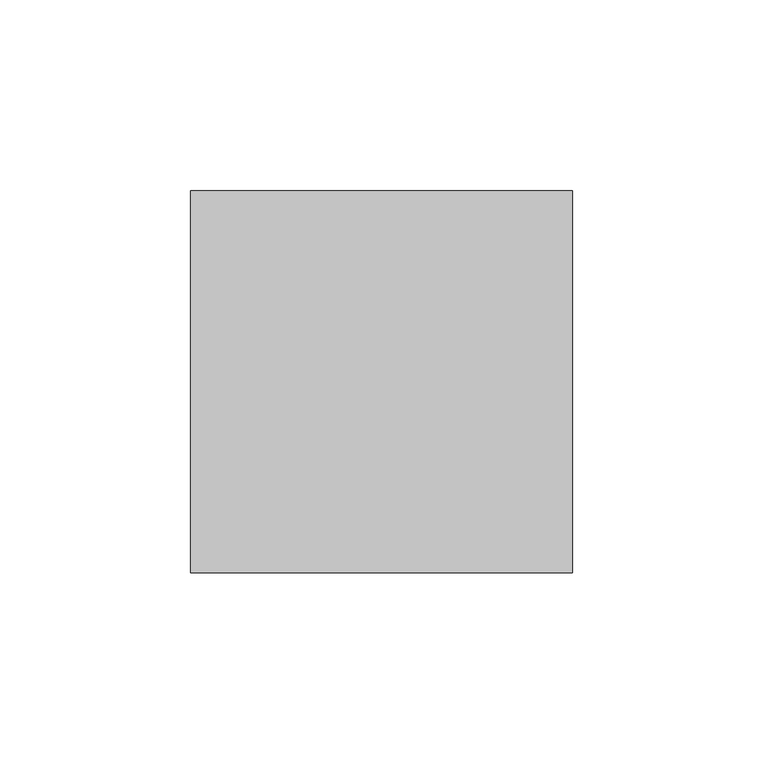
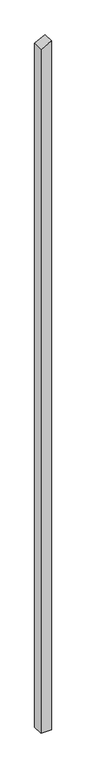
"""IFC4 building model written with IfcOpenShell, lengths in millimetres: column geometry, Holzstütze 159756 : Holzstütze 159756."""

from ifc_helpers import new_model, si_unit, frame, origin, place, context, project, spatial, polyline, outline, extrude, source, transform, mapped, element, save


def column_1855cd1a(model_context):
    return source(origin(), model_context, "Body", "SweptSolid", [
        extrude(outline(polyline([(-500.0, 157297.7593015), (-500.0, 157397.7593015), (6396.6643707, 157397.7593015), (6345.7118258, 157297.7593015), (-500.0, 157297.7593015)])), frame((0.0, 44151.7297978, 0.0), z_axis=(0.0, 1.0, 0.0), x_axis=(0.0, 0.0, 1.0)), (0.0, 0.0, 1.0), 100.0),
    ])


if __name__ == "__main__":
    model = new_model("IFC4")
    model_context = context("Model", 3, world=origin())
    ifc_project = project(units=[si_unit("LENGTHUNIT", "METRE", prefix="MILLI")], contexts=[model_context])
    site = spatial("IfcSite", under=ifc_project)
    building = spatial("IfcBuilding", under=site)
    placement = place(None, origin())
    column_shape = column_1855cd1a(model_context)
    element("IfcColumn", 1, ObjectType="Holzstütze 159756 : Holzstütze 159756", at=placement, inside=building, context=model_context, shape_type="MappedRepresentation", body=[
        mapped(column_shape, transform((0.0, 0.0, 0.0), x_axis=(1.0, 0.0, 0.0), y_axis=(0.0, 1.0, 0.0), z_axis=(0.0, 0.0, 1.0))),
    ])
    save(model, "model.ifc")

# Revit data of these elements
# Type "Holzstütze 159756 : Holzstütze 159756"
#   Abrechnungsart = "m"
#   Allright_Bauteil_ID = "0152St 0000143348"
#   Bezeichnung = "Holzstütze"
#   Codetext = "ST-HOLZ\\"
#   Gewerk = "Zimmer- und Holzbauarbeiten"
#   Material = "Holz"
#   Objektname = "Stütze"
#   NameOverride = "Holzstütze"
#   Reference = "Holzstütze"
#   Status = "NEW"
#   ThermalTransmittance = 0.0000 BTU/(h·ft²·°F)
#   Roll = 0.00°
#   Slope = 0.00°
#   2D Interaktion = yes
#   IsExternal = yes
#   LoadBearing = yes
# Element 1 (IfcColumn, "Holzstütze 159756 : Holzstütze 159756")
#   Materials on its faces: "holzschalung"
# Materials
#   "holzschalung": class "Unassigned", colour RGB 128 128 128, transparency 0
